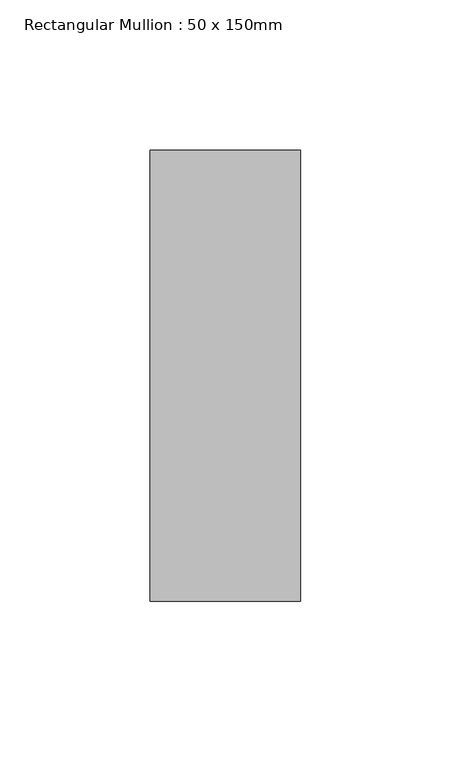
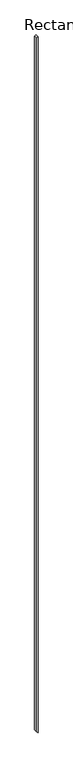
"""IFC4 building model written with IfcOpenShell, lengths in millimetres: member geometry, Rectangular Mullion : 50 x 150mm."""

from ifc_helpers import new_model, si_unit, frame, origin, place, context, project, spatial, polyline, outline, extrude, source, transform, mapped, element, save


def rectangular_mullion_50_x_150mm_3a89df96(model_context):
    return source(origin(), model_context, "Body", "SweptSolid", [
        extrude(outline(polyline([(0.0, 0.0), (-50.0, -50.0), (-30950.0, -50.0), (-31000.0, 0.0), (0.0, 0.0)])), frame((0.0, -75.0, 0.0), z_axis=(0.0, 1.0, 0.0), x_axis=(0.0, 0.0, 1.0)), (0.0, 0.0, 1.0), 150.0),
    ])


if __name__ == "__main__":
    model = new_model("IFC4")
    model_context = context("Model", 3, world=origin())
    ifc_project = project(units=[si_unit("LENGTHUNIT", "METRE", prefix="MILLI")], contexts=[model_context])
    site = spatial("IfcSite", under=ifc_project)
    building = spatial("IfcBuilding", under=site)
    placement = place(None, origin())
    rectangular_mullion_50_x_150mm_shape = rectangular_mullion_50_x_150mm_3a89df96(model_context)
    element("IfcMember", 1, ObjectType="Rectangular Mullion : 50 x 150mm", at=placement, inside=building, context=model_context, shape_type="MappedRepresentation", body=[
        mapped(rectangular_mullion_50_x_150mm_shape, transform((0.0, 0.0, 0.0), x_axis=(1.0, 0.0, 0.0), y_axis=(0.0, 1.0, 0.0), z_axis=(0.0, 0.0, 1.0))),
    ])
    save(model, "model.ifc")

# Revit data of these elements
# Type "Rectangular Mullion : 50 x 150mm"
#   built-in parameter 1007304 = 0.492126 (stored number, unit not read)
#   built-in parameter 1007301 = 0.082021 (stored number, unit not read)
#   built-in parameter 1007300 = 0.082021 (stored number, unit not read)
# Element 1 (IfcMember, "Rectangular Mullion : 50 x 150mm")
#   Materials on its faces: "Metal - Aluminium"
# Materials
#   "Metal - Aluminium": class "Metal", colour RGB 247 247 247, transparency 0
